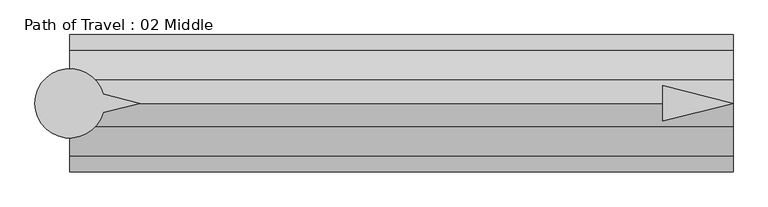
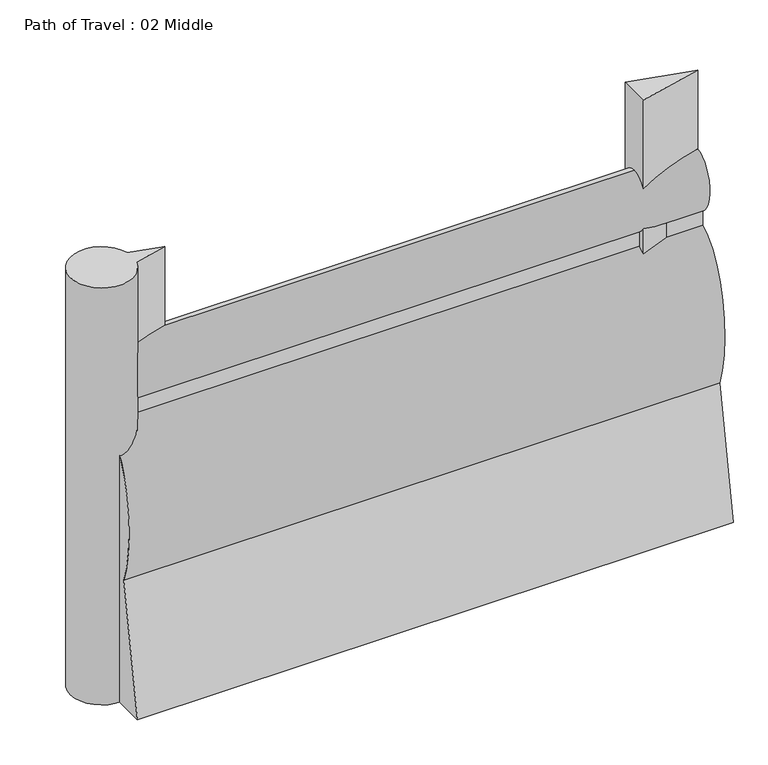
"""IFC4 building model written with IfcOpenShell, lengths in millimetres: proxy geometry, Path of Travel : 02 Middle."""

from ifc_helpers import new_model, si_unit, point, frame, frame_2d, origin, origin_with_axes, place, context, project, spatial, polyline, circle_curve, ellipse_curve, trimmed, segment, composite_curve, outline, extrude, source, transform, mapped, element, save
from ifc_brep_helpers import plane_surface, extruded_surface, advanced_brep


def path_of_travel_02_middle_62765c6b(model_context):
    return source(origin(), model_context, "Body", "SolidModel", [
        advanced_brep(
        [(227.5554837, 0.0, 1727.2), (227.5554837, 42.9018657, 1436.6534209), (227.5554837, 42.9018657, 1363.4763406), (227.5554837, 184.1186263, 643.4144547), (227.5554837, 297.5699544, 0.0), (227.5554837, 145.6574193, 0.0), (227.5554837, 0.0, 584.2), (227.5554837, -145.6574193, 0.0), (227.5554837, -297.5699544, 0.0), (227.5554837, -184.1186263, 643.4144547), (227.5554837, -42.9018657, 1363.4763406), (227.5554837, -42.9018657, 1436.6534209), (3103.4587098, 0.0, 1727.2), (3103.4587098, -42.9018657, 1436.6534209), (3103.4587098, -42.9018657, 1363.4763406), (3103.4587098, -184.1186263, 643.4144547), (3103.4587098, -297.5699544, 0.0), (3103.4587098, -145.6574193, 0.0), (3103.4587098, 0.0, 584.2), (3103.4587098, 145.6574193, 0.0), (3103.4587098, 297.5699544, 0.0), (3103.4587098, 184.1186263, 643.4144547), (3103.4587098, 42.9018657, 1363.4763406), (3103.4587098, 42.9018657, 1436.6534209)],
        [
            (0, 1, ellipse_curve(frame((227.5554837, 0.0, 1574.8), z_axis=(-1.0, 0.0, 0.0), x_axis=(0.0, 0.0, 1.0)), 152.4, 101.6)),
            (1, 2),
            (2, 3, ellipse_curve(frame((227.5554837, 0.0, 914.4), z_axis=(-1.0, 0.0, 0.0), x_axis=(0.0, 0.0, -1.0)), 457.2, 228.6)),
            (3, 4),
            (4, 5),
            (5, 6),
            (6, 7),
            (7, 8),
            (8, 9),
            (9, 10, ellipse_curve(frame((227.5554837, 0.0, 914.4), z_axis=(-1.0, 0.0, 0.0), x_axis=(0.0, 0.0, -1.0)), 457.2, 228.6)),
            (10, 11),
            (11, 0, ellipse_curve(frame((227.5554837, 0.0, 1574.8), z_axis=(-1.0, 0.0, 0.0), x_axis=(0.0, 0.0, 1.0)), 152.4, 101.6)),
            (12, 13, ellipse_curve(frame((3103.4587098, 0.0, 1574.8), z_axis=(1.0, 0.0, 0.0), x_axis=(0.0, 0.0, 1.0)), 152.4, 101.6)),
            (13, 14),
            (14, 15, ellipse_curve(frame((3103.4587098, 0.0, 914.4), z_axis=(1.0, 0.0, 0.0), x_axis=(0.0, 0.0, -1.0)), 457.2, 228.6)),
            (15, 16),
            (16, 17),
            (17, 18),
            (18, 19),
            (19, 20),
            (20, 21),
            (21, 22, ellipse_curve(frame((3103.4587098, 0.0, 914.4), z_axis=(1.0, 0.0, 0.0), x_axis=(0.0, 0.0, -1.0)), 457.2, 228.6)),
            (22, 23),
            (23, 12, ellipse_curve(frame((3103.4587098, 0.0, 1574.8), z_axis=(1.0, 0.0, 0.0), x_axis=(0.0, 0.0, 1.0)), 152.4, 101.6)),
            (0, 12),
            (23, 1),
            (22, 2),
            (21, 3),
            (20, 4),
            (19, 5),
            (18, 6),
            (17, 7),
            (16, 8),
            (15, 9),
            (14, 10),
            (13, 11),
        ],
        [
            plane_surface(frame((227.5554837, 0.0, 0.0), z_axis=(-1.0, 0.0, 0.0), x_axis=(0.0, 0.0, 1.0))),
            plane_surface(frame((3103.4587098, 0.0, 0.0), z_axis=(1.0, 0.0, 0.0), x_axis=(0.0, 0.0, 1.0))),
            extruded_surface(trimmed(ellipse_curve(frame((3103.4587098, 0.0, 1574.8), z_axis=(-1.0, 0.0, 0.0), x_axis=(0.0, 0.0, 1.0)), 152.4, 101.6), [point((3103.4587098, 0.0, 1727.2))], [point((3103.4587098, 42.9018657, 1436.6534209))], True, "CARTESIAN"), (-2875.9032261, 0.0, 0.0), 2875.9032261),
            plane_surface(frame((227.5554837, 42.9018657, 1436.6534209), z_axis=(0.0, 1.0, 0.0), x_axis=(1.0, 0.0, 0.0))),
            extruded_surface(trimmed(ellipse_curve(frame((3103.4587098, 0.0, 914.4), z_axis=(-1.0, 0.0, 0.0), x_axis=(0.0, 0.0, -1.0)), 457.2, 228.6), [point((3103.4587098, 42.9018657, 1363.4763406))], [point((3103.4587098, 184.1186263, 643.4144547))], True, "CARTESIAN"), (-2875.9032261, 0.0, 0.0), 2875.9032261),
            plane_surface(frame((227.5554837, 184.1186263, 643.4144547), z_axis=(0.0, 0.9848077530122078, 0.1736481776669322), x_axis=(1.0, 0.0, 0.0))),
            plane_surface(frame((227.5554837, 297.5699544, 0.0), z_axis=(0.0, 0.0, -1.0), x_axis=(1.0, 0.0, 0.0))),
            plane_surface(frame((227.5554837, 145.6574193, 0.0), z_axis=(0.0, -0.9702957262760199, -0.2419218955995739), x_axis=(1.0, 0.0, 0.0))),
            plane_surface(frame((227.5554837, 0.0, 584.2), z_axis=(0.0, 0.9702957262759961, -0.24192189559966923), x_axis=(1.0, 0.0, 0.0))),
            plane_surface(frame((227.5554837, -145.6574193, 0.0), z_axis=(0.0, 0.0, -1.0), x_axis=(1.0, 0.0, 0.0))),
            plane_surface(frame((227.5554837, -297.5699544, 0.0), z_axis=(0.0, -0.984807753012208, 0.17364817766693066), x_axis=(1.0, 0.0, 0.0))),
            extruded_surface(trimmed(ellipse_curve(frame((3103.4587098, 0.0, 914.4), z_axis=(-1.0, 0.0, 0.0), x_axis=(0.0, 0.0, -1.0)), 457.2, 228.6), [point((3103.4587098, -184.1186263, 643.4144547))], [point((3103.4587098, -42.9018657, 1363.4763406))], True, "CARTESIAN"), (-2875.9032261, 0.0, 0.0), 2875.9032261),
            plane_surface(frame((227.5554837, -42.9018657, 1363.4763406), z_axis=(0.0, -1.0, 0.0), x_axis=(1.0, 0.0, 0.0))),
            extruded_surface(trimmed(ellipse_curve(frame((3103.4587098, 0.0, 1574.8), z_axis=(-1.0, 0.0, 0.0), x_axis=(0.0, 0.0, 1.0)), 152.4, 101.6), [point((3103.4587098, -42.9018657, 1436.6534209))], [point((3103.4587098, 0.0, 1727.2))], True, "CARTESIAN"), (-2875.9032261, 0.0, 0.0), 2875.9032261),
        ],
        [
            (0, [[1, 2, 3, 4, 5, 6, 7, 8, 9, 10, 11, 12]]),
            (1, [[13, 14, 15, 16, 17, 18, 19, 20, 21, 22, 23, 24]]),
            (2, [[-1, 25, -24, 26]]),
            (3, [[-2, -26, -23, 27]]),
            (4, [[-3, -27, -22, 28]]),
            (5, [[-4, -28, -21, 29]]),
            (6, [[-5, -29, -20, 30]]),
            (7, [[-6, -30, -19, 31]]),
            (8, [[-7, -31, -18, 32]]),
            (9, [[-8, -32, -17, 33]]),
            (10, [[-9, -33, -16, 34]]),
            (11, [[-10, -34, -15, 35]]),
            (12, [[-11, -35, -14, 36]]),
            (13, [[-12, -36, -13, -25]]),
        ],
    ),
        extrude(outline(polyline([(2797.4535633, 76.2006338), (3103.4587098, 0.0), (2797.4535633, -76.2006338), (2797.4535633, 76.2006338)])), origin_with_axes(), (0.0, 0.0, 1.0), 2129.5973753),
        extrude(outline(composite_curve([segment(polyline([(372.7837828, 39.4440225), (531.182385, 0.0), (372.7837828, -39.4440225)]), True, "CONTINUOUS"), segment(trimmed(circle_curve(frame_2d((227.2200886, 0.0)), 150.8131956), [point((372.7837828, -39.4440225))], [point((372.7837828, 39.4440225))], False, "CARTESIAN"), True, "CONTINUOUS")], self_intersect=False)), origin_with_axes(), (0.0, 0.0, 1.0), 2129.5973753),
    ])


if __name__ == "__main__":
    model = new_model("IFC4")
    model_context = context("Model", 3, world=origin())
    ifc_project = project(units=[si_unit("LENGTHUNIT", "METRE", prefix="MILLI")], contexts=[model_context])
    site = spatial("IfcSite", under=ifc_project)
    building = spatial("IfcBuilding", under=site)
    placement = place(None, origin())
    path_of_travel_02_middle_shape = path_of_travel_02_middle_62765c6b(model_context)
    element("IfcBuildingElementProxy", 1, Name="Path of Travel : 02 Middle", ObjectType="Path of Travel : 02 Middle", at=placement, inside=building, context=model_context, shape_type="MappedRepresentation", body=[
        mapped(path_of_travel_02_middle_shape, transform((0.0, 0.0, 0.0), x_axis=(1.0, 0.0, 0.0), y_axis=(0.0, 1.0, 0.0), z_axis=(0.0, 0.0, 1.0))),
    ])
    save(model, "model.ifc")

# Revit data of these elements
# Type "Path of Travel : 02 Middle"
#   Path of Egress [instance default] = 4' - 0"
#   built-in parameter 1001306 [instance default] = 4 (stored number, unit not read)
#   Dot at Start = no
#   Arrow in Middle = yes
#   Arrow at End = no
#   Egress Path = none
# Element 1 (IfcBuildingElementProxy, "Path of Travel : 02 Middle")
#   Path of Egress = 9' - 5.22454"
#   built-in parameter 1001306 = 9.43538 (stored number, unit not read)
#   Materials on its faces: "Egress Path Solid", "solid"
# Materials
#   "Egress Path Solid": class "Unassigned", colour RGB 255 128 64, transparency 0.75, Comments = "Rendering appearance not upgraded "
#   "solid": class "Generic", colour RGB 120 120 120, transparency 0, Cost = 0
